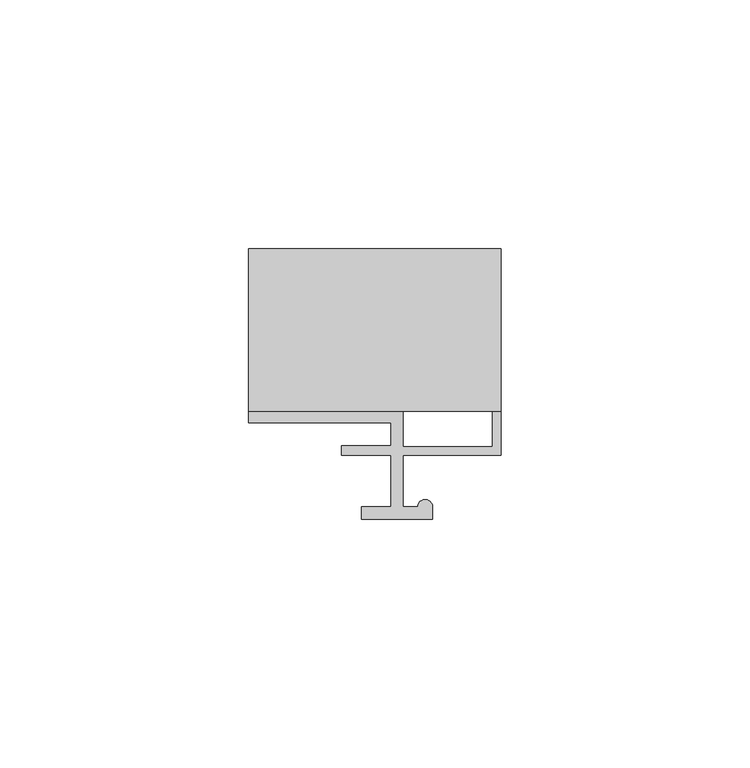
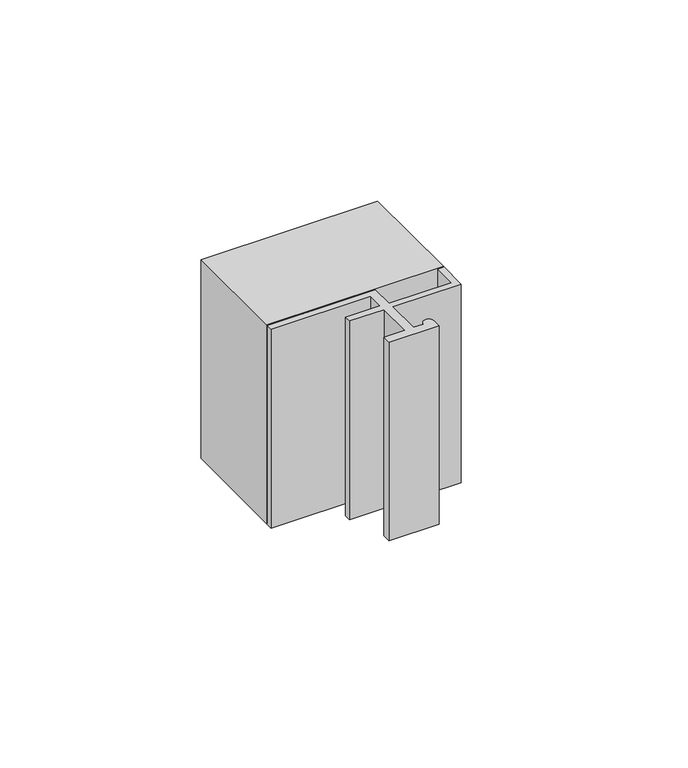
"""IFC4 building model written with IfcOpenShell, lengths in millimetres: proxy geometry, Generic Models 9:Generic Models 5:348123:Generic Models 5:348123 : Generic Models 9:Generic Models 5:348123:3 : Generic Models 9:Generic Models 5:348123:Generic Models 5:348123 : Generic Models 9:Generic Models 5:348123:301771."""

from ifc_helpers import new_model, si_unit, point, frame, frame_2d, origin, place, context, project, spatial, polyline, circle_curve, trimmed, segment, composite_curve, outline, extrude, source, transform, mapped, element, save


def generic_models_f74409b6(model_context):
    return source(origin(), model_context, "Body", "SweptSolid", [
        extrude(outline(polyline([(593279.408438, -568186.6413841), (593330.208438, -568186.6413841), (593330.208438, -568219.2983921), (593279.408438, -568219.2983921), (593279.408438, -568186.6413841)])), frame((0.0, 0.0, 6086.8701239), z_axis=(0.0, 0.0, 1.0), x_axis=(1.0, 0.0, 0.0)), (0.0, 0.0, 1.0), 60.325),
        extrude(outline(composite_curve([segment(polyline([(593310.4802827, -568228.176062), (593310.4802827, -568238.5333435), (593313.439506, -568238.5333435)]), True, "CONTINUOUS"), segment(trimmed(circle_curve(frame_2d((593314.9191176, -568238.5333435)), 1.4796117), [point((593313.439506, -568238.5333435))], [point((593316.3987293, -568238.5333435))], False, "CARTESIAN"), True, "CONTINUOUS"), segment(polyline([(593316.3987293, -568238.5333435), (593316.3987293, -568240.9993629), (593302.0958166, -568240.9993629), (593302.0958166, -568238.5333435), (593308.0142632, -568238.5333435), (593308.0142632, -568228.176062), (593298.1501856, -568228.176062), (593298.1501856, -568226.2032464), (593308.0142632, -568226.2032464), (593308.0142632, -568221.5671299), (593279.408438, -568221.5671299), (593279.408438, -568219.2983921), (593310.4802827, -568219.2983921), (593310.4802827, -568226.400528), (593328.432904, -568226.400528), (593328.432904, -568219.2983921), (593330.208438, -568219.2983921), (593330.208438, -568228.176062), (593310.4802827, -568228.176062)]), True, "CONTINUOUS")], self_intersect=False)), frame((0.0, 0.0, 6086.8701239), z_axis=(0.0, 0.0, 1.0), x_axis=(1.0, 0.0, 0.0)), (0.0, 0.0, 1.0), 60.325),
    ])


if __name__ == "__main__":
    model = new_model("IFC4")
    model_context = context("Model", 3, world=origin())
    ifc_project = project(units=[si_unit("LENGTHUNIT", "METRE", prefix="MILLI")], contexts=[model_context])
    site = spatial("IfcSite", under=ifc_project)
    building = spatial("IfcBuilding", under=site)
    placement = place(None, origin())
    generic_models_shape = generic_models_f74409b6(model_context)
    element("IfcBuildingElementProxy", 1, Name="Generic Models 9:Generic Models 5:348123:Generic Models 5:348123 : Generic Models 9:Generic Models 5:348123:3 : Generic Models 9:Generic Models 5:348123:Generic Models 5:348123 : Generic Models 9:Generic Models 5:348123:301771", ObjectType="Generic Models 9:Generic Models 5:348123:Generic Models 5:348123 : Generic Models 9:Generic Models 5:348123:3 : Generic Models 9:Generic Models 5:348123:Generic Models 5:348123 : Generic Models 9:Generic Models 5:348123:301771", at=placement, inside=building, context=model_context, shape_type="MappedRepresentation", body=[
        mapped(generic_models_shape, transform((0.0, 0.0, 0.0), x_axis=(1.0, 0.0, 0.0), y_axis=(0.0, 1.0, 0.0), z_axis=(0.0, 0.0, 1.0))),
    ])
    save(model, "model.ifc")

# Revit data of these elements
# Type "Generic Models 9:Generic Models 5:348123:Generic Models 5:348123 : Generic Models 9:Generic Models 5:348123:3 : Generic Models 9:Generic Models 5:348123:Generic Models 5:348123 : Generic Models 9:Generic Models 5:348123:301771"
#   NameOverride = "Generic Models 9:Generic Models 5:348123:Generic Models 5:348123 : Generic Models 9:Generic Models 5:348123:301771"
#   ObjectTypeOverride = "Generic Models 5:348123 : Generic Models 9:Generic Models 5:348123"
#   Reference = "Generic Models 5"
#   Tag = "301771"
# Element 1 (IfcBuildingElementProxy, "Generic Models 9:Generic Models 5:348123:Generic Models 5:348123 : Generic Models 9:Generic Models 5:348123:3 : Generic Models 9:Generic Models 5:348123:Generic Models 5:348123 : Generic Models 9:Generic Models 5:348123:301771")
#   Materials on its faces: "GALVANIZED STEEL CLIP AT EVERY SEAM IN POLYCARBONATE"
# Materials
#   "GALVANIZED STEEL CLIP AT EVERY SEAM IN POLYCARBONATE": class "Unassigned", colour RGB 120 120 120, transparency 0, Cost = 0
